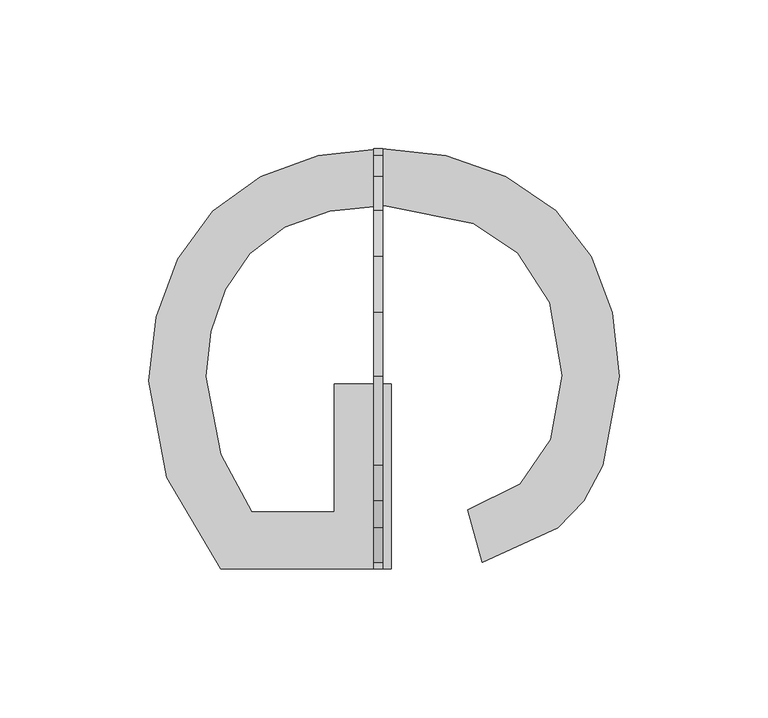
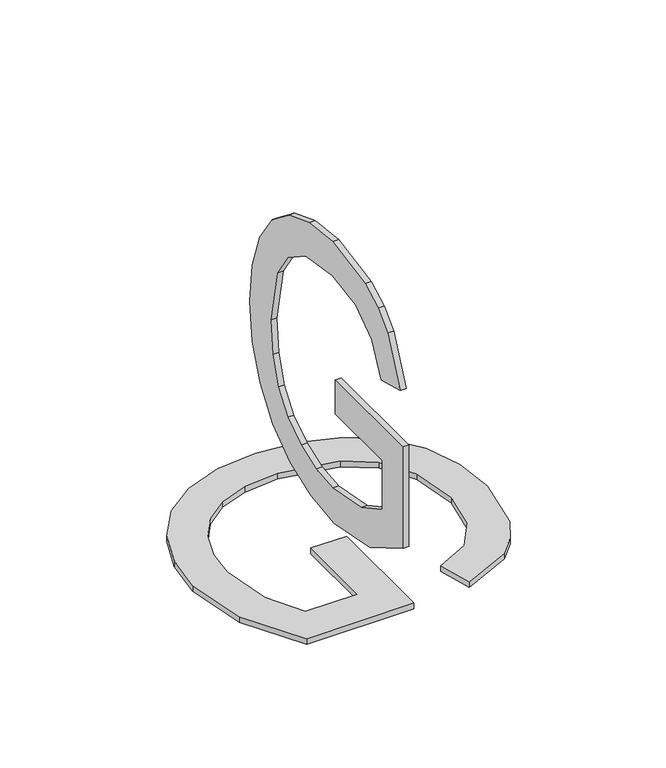
"""IFC4 building model written with IfcOpenShell, lengths in millimetres: proxy geometry, Grid Number2_FedEx : Grid Number2_FedEx."""

from ifc_helpers import new_model, si_unit, frame, origin, origin_with_axes, place, context, project, spatial, polyline, outline, extrude, source, transform, mapped, element, save


def entourage_d2fdd688(model_context):
    return source(origin(), model_context, "Body", "SweptSolid", [
        extrude(outline(polyline([(-124.4710296, 216.5403868), (-105.3341025, 216.5403868), (-105.3341025, 154.3453738), (-162.5579997, 154.3453738), (-180.6109993, 185.0504238), (-186.6660426, 217.5121839), (-184.2599104, 238.9804895), (-177.0415139, 258.3837264), (-165.2631464, 274.502476), (-149.1771015, 286.1173199), (-129.881323, 293.1394883), (-108.4737546, 295.480211), (-86.9120069, 293.1488325), (-66.8546759, 286.1546968), (-50.030439, 274.7874742), (-38.1679737, 259.3368351), (-31.1317891, 240.5176109), (-28.7863942, 219.0446331), (-34.2247201, 189.1058077), (-40.7282852, 177.1685888), (-49.3623285, 168.1187285), (-74.6851177, 156.5506056), (-79.6562336, 174.1924603), (-61.9583137, 182.9199456), (-51.7544444, 197.833293), (-47.9233213, 219.3436476), (-52.0534589, 243.844147), (-62.892734, 260.5142046), (-77.6378858, 270.3629942), (-107.6888416, 276.3432839), (-125.9894625, 274.5445249), (-141.0476452, 269.1482479), (-152.7559311, 260.3179764), (-161.0068621, 248.2172339), (-165.8985522, 234.0560947), (-167.5291155, 219.0446331), (-162.6140649, 192.8621772), (-152.1298695, 173.4823009), (-124.4710296, 173.4823009), (-124.4710296, 216.5403868)])), origin_with_axes(), (0.0, 0.0, 1.0), 3.175),
        extrude(outline(polyline([(216.5403868, 74.0411724), (173.4823009, 74.0411724), (173.4823009, 46.3823325), (192.8621772, 35.8981371), (219.0446331, 30.9830865), (234.0560947, 32.6136499), (248.2172339, 37.50534), (260.3179764, 45.7562709), (269.1482479, 57.4645569), (274.5445249, 72.5227395), (276.3432839, 90.8233604), (270.3629942, 120.8743163), (260.5142046, 135.6194681), (243.844147, 146.4587432), (219.3436476, 150.5888808), (197.833293, 146.7577577), (182.9199456, 136.5538884), (174.1924603, 118.8559685), (156.5506056, 123.8270843), (168.1187285, 149.1498736), (177.1685888, 157.7839168), (189.1058077, 164.2874819), (219.0446331, 169.7258079), (240.5176109, 167.380413), (259.3368351, 160.3442284), (274.7874742, 148.4817631), (286.1546968, 131.6575261), (293.1488325, 111.6001951), (295.480211, 90.0384474), (293.1394883, 68.6308791), (286.1173199, 49.3351006), (274.502476, 33.2490557), (258.3837264, 21.4706882), (238.9804895, 14.2522916), (217.5121839, 11.8461594), (185.0504238, 17.9012028), (154.3453738, 35.9542023), (154.3453738, 93.1780995), (216.5403868, 93.1780995), (216.5403868, 74.0411724)])), frame((-111.2489267, 0.0, 0.0), z_axis=(1.0, 0.0, 0.0), x_axis=(0.0, 1.0, 0.0)), (0.0, 0.0, 1.0), 3.175),
    ])


if __name__ == "__main__":
    model = new_model("IFC4")
    model_context = context("Model", 3, world=origin())
    ifc_project = project(units=[si_unit("LENGTHUNIT", "METRE", prefix="MILLI")], contexts=[model_context])
    site = spatial("IfcSite", under=ifc_project)
    building = spatial("IfcBuilding", under=site)
    placement = place(None, origin())
    entourage_shape = entourage_d2fdd688(model_context)
    element("IfcBuildingElementProxy", 1, Name="Grid Number2_FedEx : Grid Number2_FedEx", ObjectType="Grid Number2_FedEx : Grid Number2_FedEx", at=placement, inside=building, context=model_context, shape_type="MappedRepresentation", body=[
        mapped(entourage_shape, transform((0.0, 0.0, 0.0), x_axis=(1.0, 0.0, 0.0), y_axis=(0.0, 1.0, 0.0), z_axis=(0.0, 0.0, 1.0))),
    ])
    save(model, "model.ifc")

# Revit data of these elements
# Type "Grid Number2_FedEx : Grid Number2_FedEx"
#   Grid [instance default] = "S"
#   Label Width [instance default] = 1' - 0"
#   Half Box Width2 [instance default] = 0' - 6.13846"
#   Half Box Width [instance default] = 0' - 6"
#   Robust [instance default] = yes
#   Height = 0
#   Assembly Code = ""
# Element 1 (IfcBuildingElementProxy, "Grid Number2_FedEx : Grid Number2_FedEx")
#   Grid = "G"
#   Robust = no
#   Materials on its faces: "Letter"
# Materials
#   "Letter": class "Unassigned", colour RGB 178 187 30, transparency 0, Comments = "Rendering appearance not upgraded "
